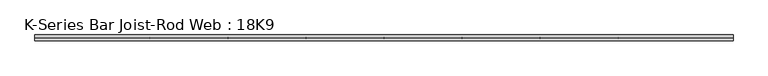
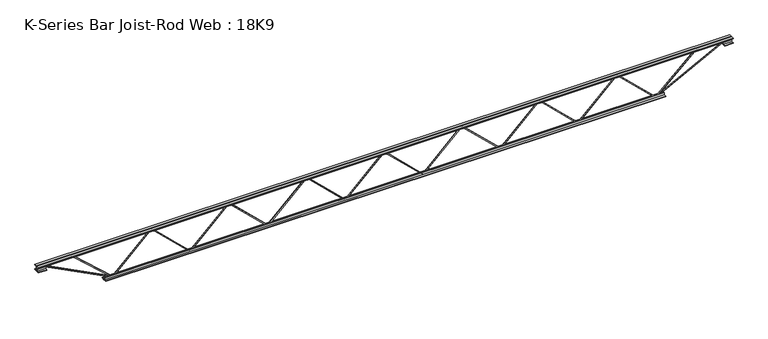
"""IFC4 building model written with IfcOpenShell, lengths in millimetres: beam geometry, K-Series Bar Joist-Rod Web : 18K9."""

from ifc_helpers import new_model, si_unit, frame, origin, place, context, project, spatial, polyline, outline, extrude, source, transform, mapped, element, save


def k_series_bar_joist_rod_web_18k9_929526b0(model_context):
    return source(origin(), model_context, "Body", "SweptSolid", [
        extrude(outline(polyline([(-217.4875, 1403.9169643), (-227.0125, 1403.9169643), (-227.0125, 1409.0121496), (217.4875, 1870.634471), (217.4875, 1873.1441004), (-227.0125, 2334.7664218), (-227.0125, 2339.8616071), (-217.4875, 2339.8616071), (-217.4875, 2338.6067925), (227.0125, 1876.984471), (227.0125, 1866.7941004), (-217.4875, 1405.171779), (-217.4875, 1403.9169643)])), frame((0.0, -4.7625, 0.0), z_axis=(0.0, 1.0, 0.0), x_axis=(0.0, 0.0, 1.0)), (0.0, 0.0, 1.0), 9.525),
        extrude(outline(polyline([(-217.4875, 467.9723214), (-227.0125, 467.9723214), (-227.0125, 473.0675068), (217.4875, 934.6898282), (217.4875, 937.1994575), (-227.0125, 1398.821779), (-227.0125, 1403.9169643), (-217.4875, 1403.9169643), (-217.4875, 1402.6621496), (227.0125, 941.0398282), (227.0125, 930.8494575), (-217.4875, 469.2271361), (-217.4875, 467.9723214)])), frame((0.0, -4.7625, 0.0), z_axis=(0.0, 1.0, 0.0), x_axis=(0.0, 0.0, 1.0)), (0.0, 0.0, 1.0), 9.525),
        extrude(outline(polyline([(-217.4875, -467.9723214), (-227.0125, -467.9723214), (-227.0125, -462.8771361), (217.4875, -1.2548147), (217.4875, 1.2548147), (-227.0125, 462.8771361), (-227.0125, 467.9723214), (-217.4875, 467.9723214), (-217.4875, 466.7175068), (227.0125, 5.0951853), (227.0125, -5.0951853), (-217.4875, -466.7175068), (-217.4875, -467.9723214)])), frame((0.0, -4.7625, 0.0), z_axis=(0.0, 1.0, 0.0), x_axis=(0.0, 0.0, 1.0)), (0.0, 0.0, 1.0), 9.525),
        extrude(outline(polyline([(-217.4875, -1403.9169643), (-227.0125, -1403.9169643), (-227.0125, -1398.821779), (217.4875, -937.1994575), (217.4875, -934.6898282), (-227.0125, -473.0675068), (-227.0125, -467.9723214), (-217.4875, -467.9723214), (-217.4875, -469.2271361), (227.0125, -930.8494575), (227.0125, -941.0398282), (-217.4875, -1402.6621496), (-217.4875, -1403.9169643)])), frame((0.0, -4.7625, 0.0), z_axis=(0.0, 1.0, 0.0), x_axis=(0.0, 0.0, 1.0)), (0.0, 0.0, 1.0), 9.525),
        extrude(outline(polyline([(-217.4875, -2339.8616071), (-227.0125, -2339.8616071), (-227.0125, -2334.7664218), (217.4875, -1873.1441004), (217.4875, -1870.634471), (-227.0125, -1409.0121496), (-227.0125, -1403.9169643), (-217.4875, -1403.9169643), (-217.4875, -1405.171779), (227.0125, -1866.7941004), (227.0125, -1876.984471), (-217.4875, -2338.6067925), (-217.4875, -2339.8616071)])), frame((0.0, -4.7625, 0.0), z_axis=(0.0, 1.0, 0.0), x_axis=(0.0, 0.0, 1.0)), (0.0, 0.0, 1.0), 9.525),
        extrude(outline(polyline([(-217.4875, 2339.8616071), (-227.0125, 2339.8616071), (-227.0125, 2344.9567925), (217.4875, 2806.5791139), (217.4875, 2809.0887432), (-227.0125, 3270.7110647), (-227.0125, 3275.80625), (-217.4875, 3275.80625), (-217.4875, 3274.5514353), (227.0125, 2812.9291139), (227.0125, 2802.7387432), (-217.4875, 2341.1164218), (-217.4875, 2339.8616071)])), frame((0.0, -4.7625, 0.0), z_axis=(0.0, 1.0, 0.0), x_axis=(0.0, 0.0, 1.0)), (0.0, 0.0, 1.0), 9.525),
        extrude(outline(polyline([(-217.4875, -3275.80625), (-227.0125, -3275.80625), (-227.0125, -3270.7110647), (217.4875, -2809.0887432), (217.4875, -2806.5791139), (-227.0125, -2344.9567925), (-227.0125, -2339.8616071), (-217.4875, -2339.8616071), (-217.4875, -2341.1164218), (227.0125, -2802.7387432), (227.0125, -2812.9291139), (-217.4875, -3274.5514353), (-217.4875, -3275.80625)])), frame((0.0, -4.7625, 0.0), z_axis=(0.0, 1.0, 0.0), x_axis=(0.0, 0.0, 1.0)), (0.0, 0.0, 1.0), 9.525),
        extrude(outline(polyline([(4.7625, 228.6), (36.5125, 228.6), (36.5125, 222.25), (11.1125, 222.25), (11.1125, 196.85), (4.7625, 196.85), (4.7625, 228.6)])), frame((-4190.20625, 0.0, 0.0), z_axis=(1.0, 0.0, 0.0), x_axis=(0.0, 1.0, 0.0)), (0.0, 0.0, 1.0), 8380.4125),
        extrude(outline(polyline([(-4.7625, 228.6), (-4.7625, 196.85), (-11.1125, 196.85), (-11.1125, 222.25), (-36.5125, 222.25), (-36.5125, 228.6), (-4.7625, 228.6)])), frame((-4190.20625, 0.0, 0.0), z_axis=(1.0, 0.0, 0.0), x_axis=(0.0, 1.0, 0.0)), (0.0, 0.0, 1.0), 8380.4125),
        extrude(outline(polyline([(-4.7625, 165.1), (-36.5125, 165.1), (-36.5125, 171.45), (-11.1125, 171.45), (-11.1125, 196.85), (-4.7625, 196.85), (-4.7625, 165.1)])), frame((-4190.20625, 0.0, 0.0), z_axis=(1.0, 0.0, 0.0), x_axis=(0.0, 1.0, 0.0)), (0.0, 0.0, 1.0), 101.6),
        extrude(outline(polyline([(36.5125, 165.1), (4.7625, 165.1), (4.7625, 196.85), (11.1125, 196.85), (11.1125, 171.45), (36.5125, 171.45), (36.5125, 165.1)])), frame((-4190.20625, 0.0, 0.0), z_axis=(1.0, 0.0, 0.0), x_axis=(0.0, 1.0, 0.0)), (0.0, 0.0, 1.0), 101.6),
        extrude(outline(polyline([(4.7625, 165.1), (4.7625, 196.85), (11.1125, 196.85), (11.1125, 171.45), (36.5125, 171.45), (36.5125, 165.1), (4.7625, 165.1)])), frame((4088.60625, 0.0, 0.0), z_axis=(1.0, 0.0, 0.0), x_axis=(0.0, 1.0, 0.0)), (0.0, 0.0, 1.0), 101.6),
        extrude(outline(polyline([(-4.7625, 165.1), (-36.5125, 165.1), (-36.5125, 171.45), (-11.1125, 171.45), (-11.1125, 196.85), (-4.7625, 196.85), (-4.7625, 165.1)])), frame((4088.60625, 0.0, 0.0), z_axis=(1.0, 0.0, 0.0), x_axis=(0.0, 1.0, 0.0)), (0.0, 0.0, 1.0), 101.6),
        extrude(outline(polyline([(4.7625, -228.6), (4.7625, -196.85), (11.1125, -196.85), (11.1125, -222.25), (36.5125, -222.25), (36.5125, -228.6), (4.7625, -228.6)])), frame((-3377.40625, 0.0, 0.0), z_axis=(1.0, 0.0, 0.0), x_axis=(0.0, 1.0, 0.0)), (0.0, 0.0, 1.0), 6754.8125),
        extrude(outline(polyline([(-4.7625, -228.6), (-36.5125, -228.6), (-36.5125, -222.25), (-11.1125, -222.25), (-11.1125, -196.85), (-4.7625, -196.85), (-4.7625, -228.6)])), frame((-3377.40625, 0.0, 0.0), z_axis=(1.0, 0.0, 0.0), x_axis=(0.0, 1.0, 0.0)), (0.0, 0.0, 1.0), 6754.8125),
        extrude(outline(polyline([(0.0, -9.525), (0.0, 0.0), (914.4881902, 0.0), (914.4881902, -9.525), (0.0, -9.525)])), frame((-4090.788852, 4.7625, 192.6170749), z_axis=(0.45828913319472714, 0.0, 0.8888031674086371), x_axis=(0.8888031674086371, 0.0, -0.45828913319472714)), (0.0, 0.0, 1.0), 9.525),
        extrude(outline(polyline([(0.0, -9.525), (0.0, 0.0), (628.2060996, 0.0), (628.2060996, -9.525), (0.0, -9.525)])), frame((-3746.9558149, 4.7625, 193.30225), z_axis=(0.6671377438724063, 0.0, 0.7449343801307842), x_axis=(0.7449343801307842, 0.0, -0.6671377438724063)), (0.0, 0.0, 1.0), 9.525),
        extrude(outline(polyline([(0.0, -9.525), (0.0, 0.0), (914.4881902, 0.0), (914.4881902, -9.525), (0.0, -9.525)])), frame((4090.788852, -4.7625, 192.6170749), z_axis=(-0.4582891331947151, 0.0, 0.8888031674086433), x_axis=(-0.8888031674086433, 0.0, -0.4582891331947151)), (0.0, 0.0, 1.0), 9.525),
        extrude(outline(polyline([(0.0, -9.525), (0.0, 0.0), (628.2060996, 0.0), (628.2060996, -9.525), (0.0, -9.525)])), frame((3746.9558149, -4.7625, 193.30225), z_axis=(-0.6671377438724027, 0.0, 0.7449343801307874), x_axis=(-0.7449343801307874, 0.0, -0.6671377438724027)), (0.0, 0.0, 1.0), 9.525),
    ])


if __name__ == "__main__":
    model = new_model("IFC4")
    model_context = context("Model", 3, world=origin())
    ifc_project = project(units=[si_unit("LENGTHUNIT", "METRE", prefix="MILLI")], contexts=[model_context])
    site = spatial("IfcSite", under=ifc_project)
    building = spatial("IfcBuilding", under=site)
    placement = place(None, origin())
    k_series_bar_joist_rod_web_18k9_shape = k_series_bar_joist_rod_web_18k9_929526b0(model_context)
    element("IfcBeam", 1, ObjectType="K-Series Bar Joist-Rod Web : 18K9", at=placement, inside=building, context=model_context, shape_type="MappedRepresentation", body=[
        mapped(k_series_bar_joist_rod_web_18k9_shape, transform((0.0, 0.0, 0.0), x_axis=(1.0, 0.0, 0.0), y_axis=(0.0, 1.0, 0.0), z_axis=(0.0, 0.0, 1.0))),
    ])
    save(model, "model.ifc")

# Revit data of these elements
# Type "K-Series Bar Joist-Rod Web : 18K9"
#   Assembly Code = "B1010350"
#   Wt = 10.2
#   Web Thickness = 0' - 0 3/8"
#   Start Offset [instance default] = 0' - 0"
#   Start Extension [instance default] = 0' - 0"
#   Seat Length = 0' - 4"
#   Seat Depth = 0' - 2 1/2"
#   PanelArrayLength [instance default] = 18' - 0"
#   Panel [instance default] = 3' - 0"
#   End Offset [instance default] = 0' - 0"
#   End Extension [instance default] = 0' - 0"
#   End Panel = 3' - 0"
#   Cord Leg = 0' - 1 1/4"
#   Chord Thickness = 0' - 0 1/4"
#   Length [instance default] = 24' - 0"
#   Depth = 1' - 6"
#   PanelArrayNum [instance default] = 6
#   Structural Material = none
# Element 1 (IfcBeam, "K-Series Bar Joist-Rod Web : 18K9")
#   PanelArrayLength = 21' - 5 15/16"
#   Panel = 3' - 0.84821"
#   PanelArrayNum = 7
